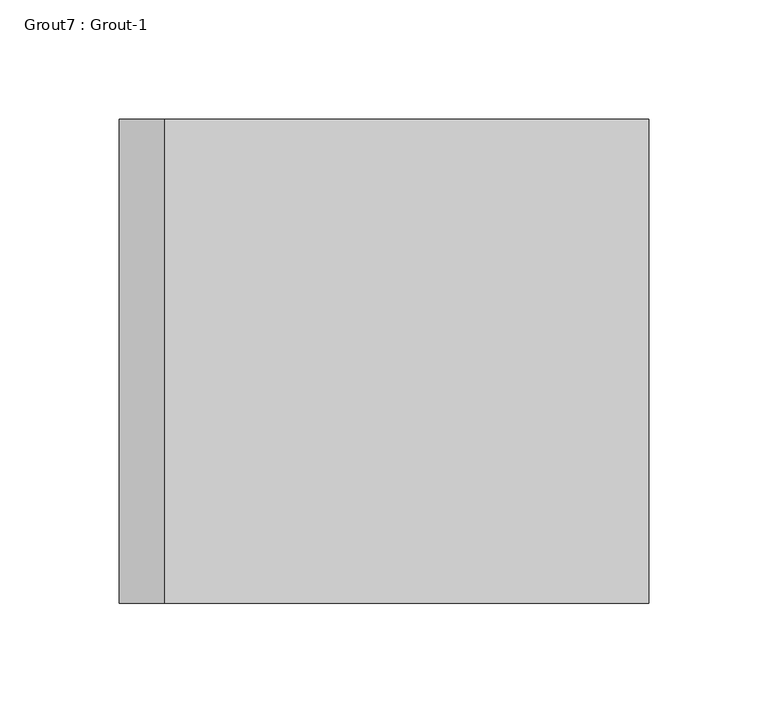
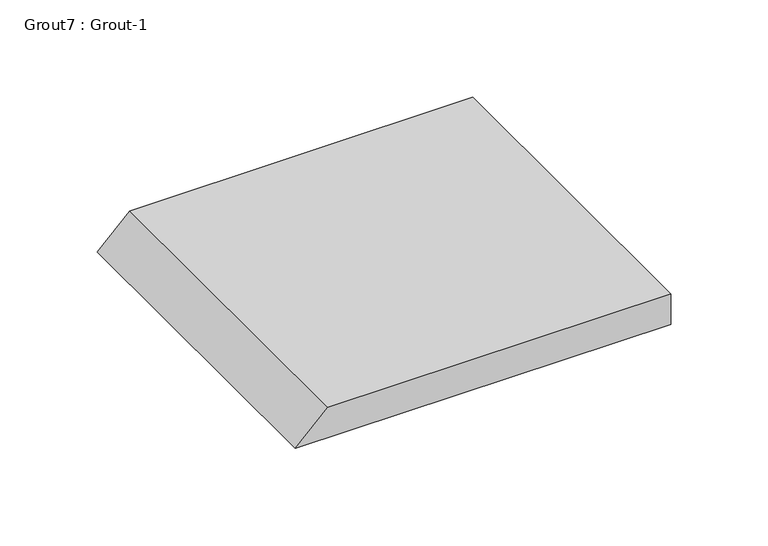
"""IFC4 building model written with IfcOpenShell, lengths in millimetres: proxy geometry, Grout7 : Grout-1."""

from ifc_helpers import new_model, si_unit, frame, origin, place, context, project, spatial, polyline, outline, extrude, source, transform, mapped, element, save


def grout7_grout_1_248e8b60(model_context):
    return source(origin(), model_context, "Body", "SweptSolid", [
        extrude(outline(polyline([(19.05, 590115.4434739), (0.0, 590096.3934739), (0.0, 590318.6434739), (19.05, 590318.6434739), (19.05, 590115.4434739)])), frame((0.0, -536468.3913841, 0.0), z_axis=(0.0, 1.0, 0.0), x_axis=(0.0, 0.0, 1.0)), (0.0, 0.0, 1.0), 203.2),
    ])


if __name__ == "__main__":
    model = new_model("IFC4")
    model_context = context("Model", 3, world=origin())
    ifc_project = project(units=[si_unit("LENGTHUNIT", "METRE", prefix="MILLI")], contexts=[model_context])
    site = spatial("IfcSite", under=ifc_project)
    building = spatial("IfcBuilding", under=site)
    placement = place(None, origin())
    grout7_grout_1_shape = grout7_grout_1_248e8b60(model_context)
    element("IfcBuildingElementProxy", 1, Name="Grout7 : Grout-1", ObjectType="Grout7 : Grout-1", at=placement, inside=building, context=model_context, shape_type="MappedRepresentation", body=[
        mapped(grout7_grout_1_shape, transform((0.0, 0.0, 0.0), x_axis=(1.0, 0.0, 0.0), y_axis=(0.0, 1.0, 0.0), z_axis=(0.0, 0.0, 1.0))),
    ])
    save(model, "model.ifc")

# Revit data of these elements
# Element 1 (IfcBuildingElementProxy, "Grout7 : Grout-1")
#   Materials on its faces: "3/4\" NON SHRINK GROUT"
# Materials
#   "3/4\" NON SHRINK GROUT": class "Generic", colour RGB 145 145 143, transparency 0, Cost = 0
